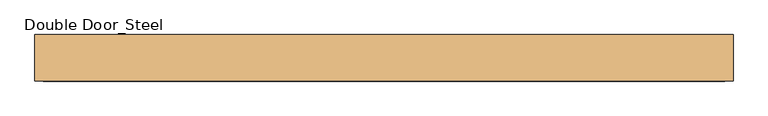
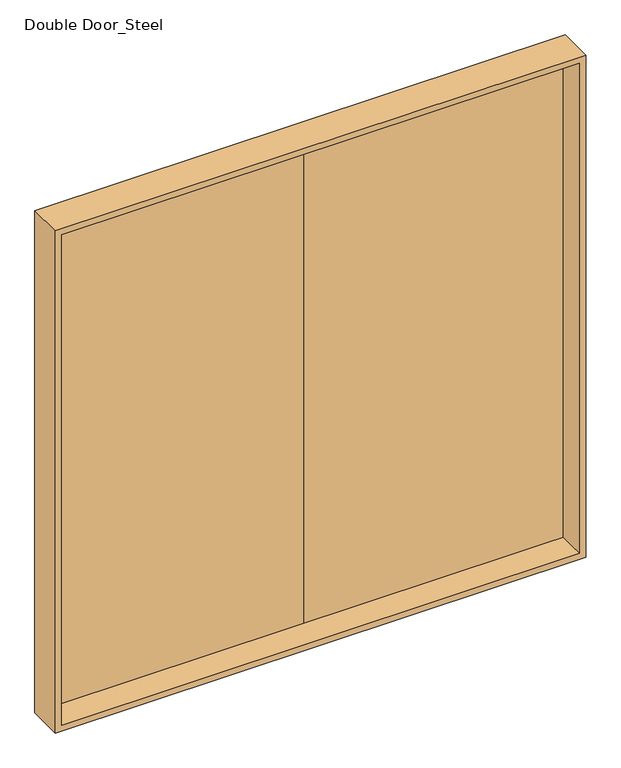
"""IFC4 building model written with IfcOpenShell, lengths in millimetres: door geometry, Double Door_Steel : H_DR_AR_B12_Double Door_Steel_W3000xH3000."""

from ifc_helpers import new_model, si_unit, frame, origin, place, context, project, spatial, polyline, outline, extrude, faceted_brep, source, transform, mapped, element, save


def double_door_steel_ab4802d0(model_context):
    return source(origin(), model_context, "Body", "SolidModel", [
        extrude(outline(polyline([(1480.0, 60.0), (0.0, 60.0), (0.0, 100.0), (1480.0, 100.0), (1480.0, 60.0)])), frame((0.0, 0.0, 20.0), z_axis=(0.0, 0.0, 1.0), x_axis=(1.0, 0.0, 0.0)), (0.0, 0.0, 1.0), 2960.0),
        extrude(outline(polyline([(0.0, 60.0), (-1480.0, 60.0), (-1480.0, 100.0), (0.0, 100.0), (0.0, 60.0)])), frame((0.0, 0.0, 20.0), z_axis=(0.0, 0.0, 1.0), x_axis=(1.0, 0.0, 0.0)), (0.0, 0.0, 1.0), 2960.0),
        faceted_brep([(1500.0, -100.0, 3000.0), (1500.0, 100.0, 3000.0), (-1500.0, 100.0, 3000.0), (-1500.0, -100.0, 3000.0), (1465.0, 60.0, 2965.0), (1465.0, -100.0, 2965.0), (-1465.0, -100.0, 2965.0), (-1465.0, 60.0, 2965.0), (1480.0, 100.0, 2980.0), (1480.0, 60.0, 2980.0), (-1480.0, 60.0, 2980.0), (-1480.0, 100.0, 2980.0), (-1500.0, 100.0, 0.0), (-1500.0, -100.0, 0.0), (-1465.0, -100.0, 35.0), (-1465.0, 60.0, 35.0), (-1480.0, 60.0, 20.0), (-1480.0, 100.0, 20.0), (1500.0, 100.0, 0.0), (1480.0, 100.0, 20.0), (1500.0, -100.0, 0.0), (1465.0, -100.0, 35.0), (1465.0, 60.0, 35.0), (1480.0, 60.0, 20.0)], [[[0, 1, 2, 3]], [[4, 5, 6, 7]], [[8, 9, 10, 11]], [[3, 2, 12, 13]], [[7, 6, 14, 15]], [[11, 10, 16, 17]], [[18, 12, 2, 1], [8, 11, 17, 19]], [[13, 12, 18, 20]], [[0, 3, 13, 20], [21, 14, 6, 5]], [[15, 14, 21, 22]], [[23, 16, 10, 9], [4, 7, 15, 22]], [[17, 16, 23, 19]], [[20, 18, 1, 0]], [[22, 21, 5, 4]], [[19, 23, 9, 8]]]),
    ])


if __name__ == "__main__":
    model = new_model("IFC4")
    model_context = context("Model", 3, world=origin())
    ifc_project = project(units=[si_unit("LENGTHUNIT", "METRE", prefix="MILLI")], contexts=[model_context])
    site = spatial("IfcSite", under=ifc_project)
    building = spatial("IfcBuilding", under=site)
    placement = place(None, origin())
    double_door_steel_shape = double_door_steel_ab4802d0(model_context)
    element("IfcDoor", 1, ObjectType="Double Door_Steel : H_DR_AR_B12_Double Door_Steel_W3000xH3000", at=placement, inside=building, context=model_context, shape_type="MappedRepresentation", body=[
        mapped(double_door_steel_shape, transform((0.0, 0.0, 0.0), x_axis=(1.0, 0.0, 0.0), y_axis=(0.0, 1.0, 0.0), z_axis=(0.0, 0.0, 1.0))),
    ])
    save(model, "model.ifc")

# Revit data of these elements
# Type "Double Door_Steel : H_DR_AR_B12_Double Door_Steel_W3000xH3000"
#   Type Mark = "430"
#   프레임 = ""
#   철물 = ""
#   유리/마감 = ""
#   위치/개소 = ""
#   부호 = "1/SD"
#   문번호 = ""
#   문기호 = "SD"
#   Analytic Construction = "<None>"
#   Height = 3000 mm
#   Width = 3000 mm
#   Define Thermal Properties by = 1
#   문 틀 = none
#   문 = none
#   Function = (empty or 0)
#   Assembly Code = ""
#   Wall Closure = (empty or 0)
